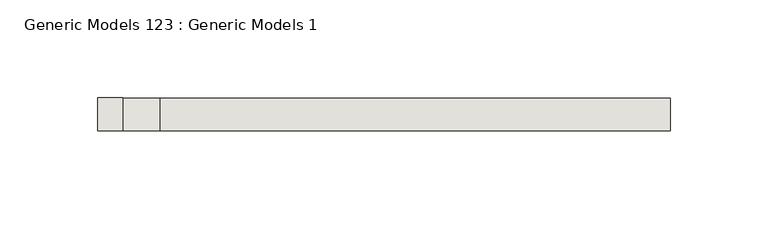
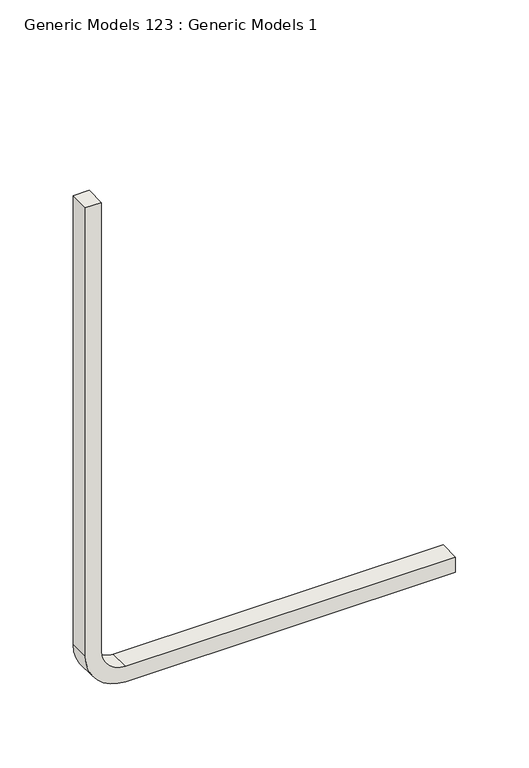
"""IFC4 building model written with IfcOpenShell, lengths in millimetres: wall geometry, Generic Models 123 : Generic Models 1."""

from ifc_helpers import new_model, si_unit, point, frame, frame_2d, origin, place, context, project, spatial, polyline, circle_curve, trimmed, segment, composite_curve, outline, extrude, source, transform, mapped, element, save


def generic_models_123_generic_models_1_7279ad26(model_context):
    return source(origin(), model_context, "Body", "SweptSolid", [
        extrude(outline(composite_curve([segment(trimmed(circle_curve(frame_2d((2490.3792423, 373565.3011146)), 31.75), [point((2490.3792423, 373533.5511146))], [point((2458.6292423, 373565.3011146))], False, "CARTESIAN"), True, "CONTINUOUS"), segment(polyline([(2458.6292423, 373565.3011146), (2458.6292423, 373825.6511146), (2471.3292423, 373825.6511146), (2471.3292423, 373565.3011146)]), True, "CONTINUOUS"), segment(trimmed(circle_curve(frame_2d((2490.3792423, 373565.3011146)), 19.05), [point((2471.3292423, 373565.3011146))], [point((2490.3792423, 373546.2511146))], True, "CARTESIAN"), True, "CONTINUOUS"), segment(polyline([(2490.3792423, 373546.2511146), (2865.0292423, 373546.2511146), (2865.0292423, 373533.5511146), (2490.3792423, 373533.5511146)]), True, "CONTINUOUS")], self_intersect=False)), frame((0.0, 407.5533734, 0.0), z_axis=(0.0, 1.0, 0.0), x_axis=(0.0, 0.0, 1.0)), (0.0, 0.0, 1.0), 16.7191266),
    ])


if __name__ == "__main__":
    model = new_model("IFC4")
    model_context = context("Model", 3, world=origin())
    ifc_project = project(units=[si_unit("LENGTHUNIT", "METRE", prefix="MILLI")], contexts=[model_context])
    site = spatial("IfcSite", under=ifc_project)
    building = spatial("IfcBuilding", under=site)
    placement = place(None, origin())
    generic_models_123_generic_models_1_shape = generic_models_123_generic_models_1_7279ad26(model_context)
    element("IfcWall", 1, ObjectType="Generic Models 123 : Generic Models 1", at=placement, inside=building, context=model_context, shape_type="MappedRepresentation", body=[
        mapped(generic_models_123_generic_models_1_shape, transform((0.0, 0.0, 0.0), x_axis=(1.0, 0.0, 0.0), y_axis=(0.0, 1.0, 0.0), z_axis=(0.0, 0.0, 1.0))),
    ])
    save(model, "model.ifc")

# Revit data of these elements
# Element 1 (IfcWall, "Generic Models 123 : Generic Models 1")
#   Materials on its faces: "#3 J's @ 24\" O.C."
# Materials
#   "#3 J's @ 24\" O.C.": class "Generic", colour RGB 255 255 255, transparency 0, Cost = 0
